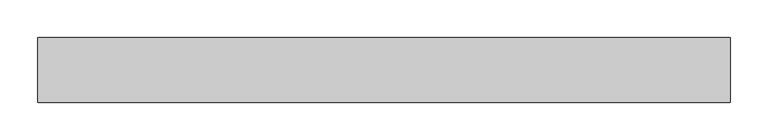
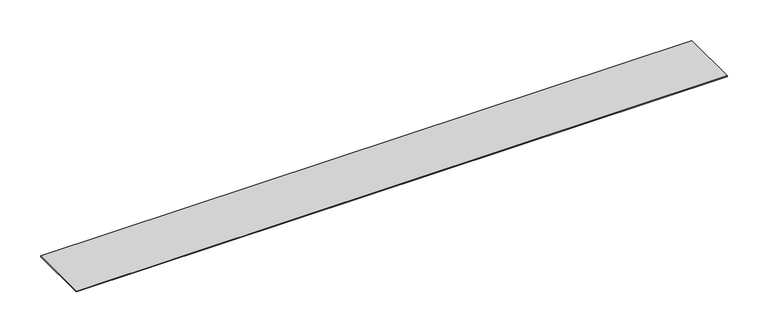
"""IFC4 building model written with IfcOpenShell, lengths in millimetres: proxy geometry, Generic Models 6:Generic Models 2:318829:Generic Models 2:318829 : Generic Models 6:Generic Models 2:318829:22 : Generic Models 6:Generic Models 2:318829:Generic Models 2:318829 : Generic Models 6:Generic Models 2:318829:300683."""

from ifc_helpers import new_model, si_unit, frame, origin, place, context, project, spatial, polyline, outline, extrude, source, transform, mapped, element, save


def generic_models_66fd3eed(model_context):
    return source(origin(), model_context, "Body", "SweptSolid", [
        extrude(outline(polyline([(593679.9536635, -579002.9006209), (593679.9536635, -579089.5913841), (592758.9138536, -579089.5913841), (592758.9138536, -579002.9006209), (593679.9536635, -579002.9006209)])), frame((0.0, 0.0, 25.4258371), z_axis=(0.0, 0.0, 1.0), x_axis=(1.0, 0.0, 0.0)), (0.0, 0.0, 1.0), 1.4049011),
    ])


if __name__ == "__main__":
    model = new_model("IFC4")
    model_context = context("Model", 3, world=origin())
    ifc_project = project(units=[si_unit("LENGTHUNIT", "METRE", prefix="MILLI")], contexts=[model_context])
    site = spatial("IfcSite", under=ifc_project)
    building = spatial("IfcBuilding", under=site)
    placement = place(None, origin())
    generic_models_shape = generic_models_66fd3eed(model_context)
    element("IfcBuildingElementProxy", 1, Name="Generic Models 6:Generic Models 2:318829:Generic Models 2:318829 : Generic Models 6:Generic Models 2:318829:22 : Generic Models 6:Generic Models 2:318829:Generic Models 2:318829 : Generic Models 6:Generic Models 2:318829:300683", ObjectType="Generic Models 6:Generic Models 2:318829:Generic Models 2:318829 : Generic Models 6:Generic Models 2:318829:22 : Generic Models 6:Generic Models 2:318829:Generic Models 2:318829 : Generic Models 6:Generic Models 2:318829:300683", at=placement, inside=building, context=model_context, shape_type="MappedRepresentation", body=[
        mapped(generic_models_shape, transform((0.0, 0.0, 0.0), x_axis=(1.0, 0.0, 0.0), y_axis=(0.0, 1.0, 0.0), z_axis=(0.0, 0.0, 1.0))),
    ])
    save(model, "model.ifc")

# Revit data of these elements
# Type "Generic Models 6:Generic Models 2:318829:Generic Models 2:318829 : Generic Models 6:Generic Models 2:318829:22 : Generic Models 6:Generic Models 2:318829:Generic Models 2:318829 : Generic Models 6:Generic Models 2:318829:300683"
#   NameOverride = "Generic Models 6:Generic Models 2:318829:Generic Models 2:318829 : Generic Models 6:Generic Models 2:318829:300683"
#   ObjectTypeOverride = "Generic Models 2:318829 : Generic Models 6:Generic Models 2:318829"
#   Reference = "Generic Models 2"
#   Tag = "300683"
# Element 1 (IfcBuildingElementProxy, "Generic Models 6:Generic Models 2:318829:Generic Models 2:318829 : Generic Models 6:Generic Models 2:318829:22 : Generic Models 6:Generic Models 2:318829:Generic Models 2:318829 : Generic Models 6:Generic Models 2:318829:300683")
#   Materials on its faces: "COMPRESSIBE THERMAL GASKET SANDWICHED BETWEEN METAL COMPONENTS"
# Materials
#   "COMPRESSIBE THERMAL GASKET SANDWICHED BETWEEN METAL COMPONENTS": class "Unassigned", colour RGB 58 208 21, transparency 0, Cost = 0
